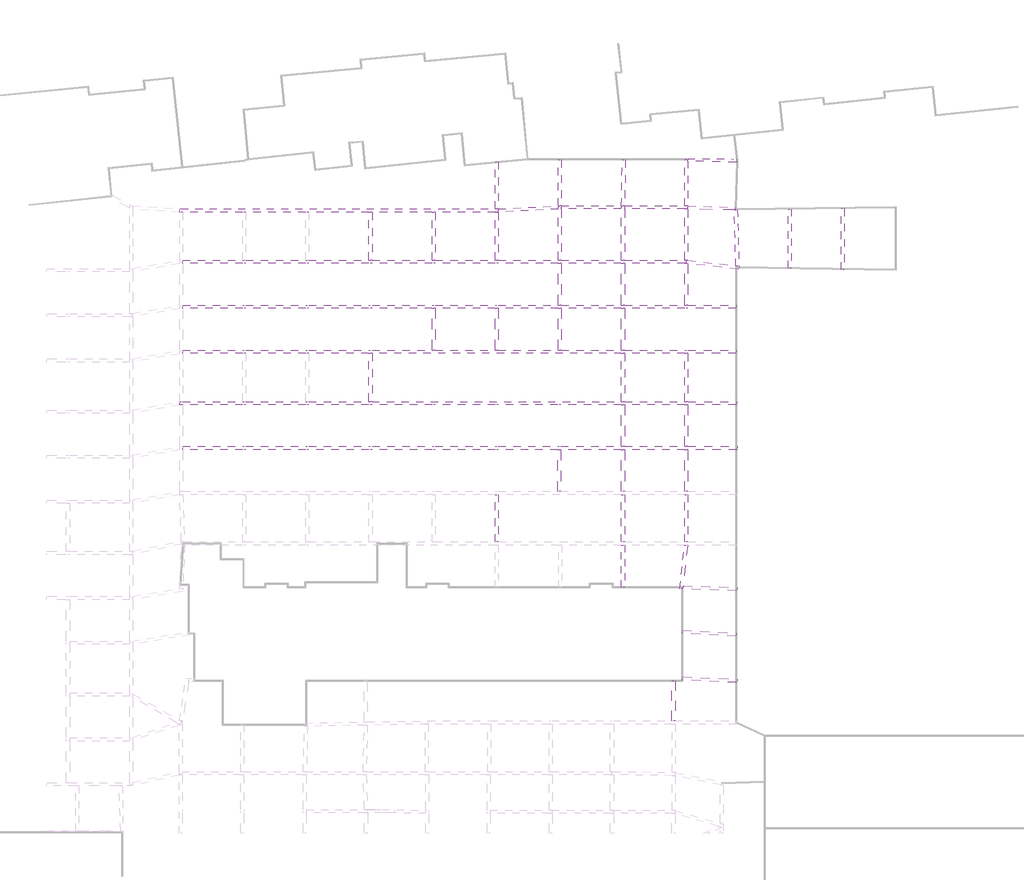
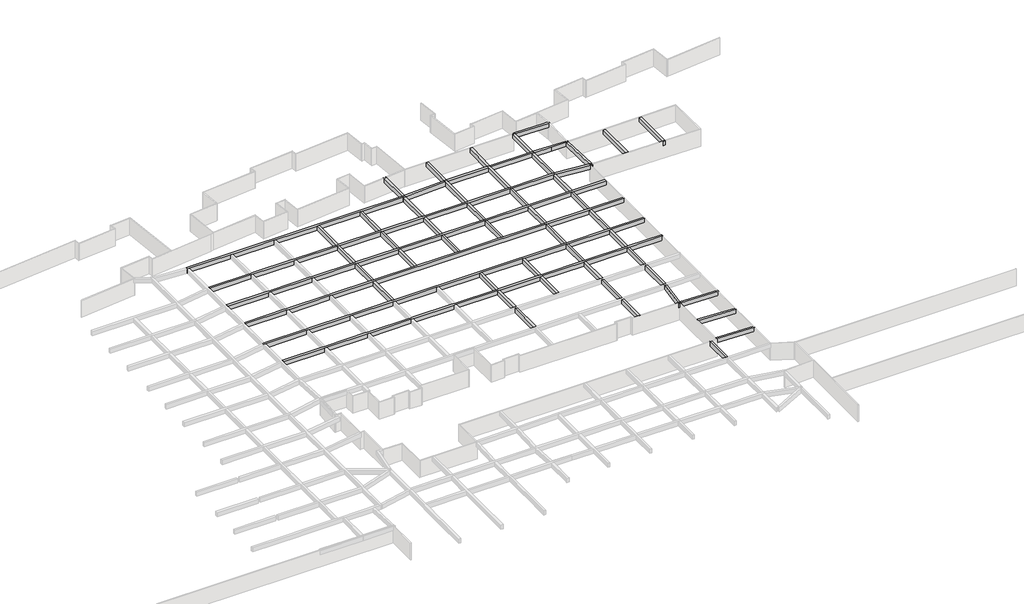
# One storey, part 20 of 20: 49 beams.
"""IFC4 building model written with IfcOpenShell, lengths in millimetres."""

import ifcopenshell
import ifcopenshell.guid

model = None  # the IFC model being written
_history = None  # IfcOwnerHistory: only IFC2X3 demands one
_inside = {}  # id of a spatial element -> (the spatial element, [elements in it])
_under = {}  # id of a project, library or spatial element -> (it, [spatial elements below it])
_declared = {}  # id of a project -> (the project, [libraries it declares])
_typed = {}  # id of a type object -> (the type object, [elements of that type])
_made_of = {}  # id of a material, layer set ... -> (it, [elements and type objects made of it])


def new_model(schema):
    """Start an empty IFC model of exactly this schema.

    Asked for "IFC4X3", IfcOpenShell would pick the latest addendum, in which some entities
    have other attributes; the version numbers below select the first issue.
    IFC2X3 requires an IfcOwnerHistory on every rooted entity: one is made here for all.
    """
    global model, _history
    if schema == "IFC4X3":
        model = ifcopenshell.file(schema_version=(4, 3, 0, 0))
    else:
        model = ifcopenshell.file(schema=schema)
    _inside.clear()
    _under.clear()
    _declared.clear()
    _typed.clear()
    _made_of.clear()
    _history = None
    if model.schema == "IFC2X3":
        org = make("IfcOrganization", Name="unknown")
        user = make(
            "IfcPersonAndOrganization",
            ThePerson=make("IfcPerson", FamilyName="unknown"),
            TheOrganization=org,
        )
        app = make(
            "IfcApplication",
            ApplicationDeveloper=org,
            Version="unknown",
            ApplicationFullName="unknown",
            ApplicationIdentifier="unknown",
        )
        _history = make(
            "IfcOwnerHistory",
            OwningUser=user,
            OwningApplication=app,
            ChangeAction="ADDED",
            CreationDate=0,
        )
    return model


def make(cls, **values):
    """One entity of the class cls with the attributes given. An attribute that is None is left unset."""
    return model.create_entity(
        cls, **{name: value for name, value in values.items() if value is not None}
    )


def rooted(cls, **values):
    """An entity with a GlobalId (a new one), such as an element, a storey or a relation."""
    return make(cls, GlobalId=ifcopenshell.guid.new(), OwnerHistory=_history, **values)


def si_unit(unit_type, name, prefix=None):
    """IfcSIUnit, for example si_unit("LENGTHUNIT", "METRE", prefix="MILLI")."""
    return make("IfcSIUnit", UnitType=unit_type, Prefix=prefix, Name=name)


def assignment(units):
    """IfcUnitAssignment: the units of a project."""
    return None if units is None else make("IfcUnitAssignment", Units=units)


def point(xyz):
    """IfcCartesianPoint."""
    return None if xyz is None else make("IfcCartesianPoint", Coordinates=xyz)


def direction(xyz):
    """IfcDirection."""
    return None if xyz is None else make("IfcDirection", DirectionRatios=xyz)


def frame(location, z_axis=None, x_axis=None):
    """IfcAxis2Placement3D, a coordinate frame: its origin and axes. An axis left out is left unset."""
    return make(
        "IfcAxis2Placement3D",
        Location=point(location),
        Axis=direction(z_axis),
        RefDirection=direction(x_axis),
    )


def origin():
    """The frame at (0, 0, 0) with its axes left unset."""
    return frame((0.0, 0.0, 0.0))


def place(relative_to, where):
    """IfcLocalPlacement: puts the frame where relative to a parent placement (None: the world)."""
    return make(
        "IfcLocalPlacement", PlacementRelTo=relative_to, RelativePlacement=where
    )


def context(
    kind, dimensions, precision=None, world=None, true_north=None, identifier=None
):
    """IfcGeometricRepresentationContext, for example the 3D "Model" context."""
    return make(
        "IfcGeometricRepresentationContext",
        ContextIdentifier=identifier,
        ContextType=kind,
        CoordinateSpaceDimension=dimensions,
        Precision=precision,
        WorldCoordinateSystem=world,
        TrueNorth=true_north,
    )


def project(units=None, contexts=None):
    """IfcProject with its units and contexts."""
    return rooted(
        "IfcProject",
        Name="project",
        RepresentationContexts=contexts,
        UnitsInContext=assignment(units),
    )


def spatial(cls, under=None, at=None, **own):
    """A site, building, storey or space (cls), placed at a placement, below another one or the project."""
    s = rooted(cls, ObjectPlacement=at, **own)
    if under is not None:
        _under.setdefault(under.id(), (under, []))[1].append(s)
    return s


def polyline(points):
    """IfcPolyline through the points."""
    return make("IfcPolyline", Points=[point(p) for p in points])


def outline(outer, holes=None, kind="AREA"):
    """IfcArbitraryClosedProfileDef: a profile drawn as a closed curve; with holes, ...WithVoids."""
    if holes is None:
        return make("IfcArbitraryClosedProfileDef", ProfileType=kind, OuterCurve=outer)
    return make(
        "IfcArbitraryProfileDefWithVoids",
        ProfileType=kind,
        OuterCurve=outer,
        InnerCurves=holes,
    )


def extrude(swept, where, along, depth):
    """IfcExtrudedAreaSolid: the profile swept, set in the frame where, extruded along a direction by depth."""
    return make(
        "IfcExtrudedAreaSolid",
        SweptArea=swept,
        Position=where,
        ExtrudedDirection=direction(along),
        Depth=depth,
    )


def faces_of(points, faces, orient=None, outer=None):
    """IfcFace entities. A face is a list of loops; a loop is a list of indices into points, from 0.

    orient and outer hold one flag for each loop. By default every Orientation is true, the
    first loop of a face is its IfcFaceOuterBound and the others are IfcFaceBound.
    """
    made = []
    for i, loops in enumerate(faces):
        bounds = []
        for j, loop in enumerate(loops):
            is_outer = j == 0 if outer is None else outer[i][j]
            bounds.append(
                make(
                    "IfcFaceOuterBound" if is_outer else "IfcFaceBound",
                    Bound=make("IfcPolyLoop", Polygon=[points[k] for k in loop]),
                    Orientation=True if orient is None else orient[i][j],
                )
            )
        made.append(make("IfcFace", Bounds=bounds))
    return made


def faceted_brep(points, faces, orient=None, outer=None, voids=None):
    """IfcFacetedBrep: a solid bounded by flat faces; with voids (closed shells), ...WithVoids."""
    shared = [point(p) for p in points]
    hull = make("IfcClosedShell", CfsFaces=faces_of(shared, faces, orient, outer))
    if voids is None:
        return make("IfcFacetedBrep", Outer=hull)
    return make(
        "IfcFacetedBrepWithVoids",
        Outer=hull,
        Voids=[
            make(cls, CfsFaces=faces_of(shared, fs, o, b)) for cls, fs, o, b in voids
        ],
    )


def shape(context_of_items, identifier, shape_type, items):
    """IfcShapeRepresentation: the items that make up one representation, for example the "Body"."""
    return make(
        "IfcShapeRepresentation",
        ContextOfItems=context_of_items,
        RepresentationIdentifier=identifier,
        RepresentationType=shape_type,
        Items=items,
    )


def source(mapping_origin, context_of_items, identifier, shape_type, items):
    """IfcRepresentationMap: a shape defined once, which mapped items show again and again."""
    return make(
        "IfcRepresentationMap",
        MappingOrigin=mapping_origin,
        MappedRepresentation=shape(context_of_items, identifier, shape_type, items),
    )


def transform(
    local_origin,
    x_axis=None,
    y_axis=None,
    z_axis=None,
    scale=None,
    scale2=None,
    scale3=None,
    uniform=True,
):
    """IfcCartesianTransformationOperator3D, or its non-uniform kind. x_axis, y_axis, z_axis: its Axis1, 2, 3."""
    if uniform:
        return make(
            "IfcCartesianTransformationOperator3D",
            Axis1=direction(x_axis),
            Axis2=direction(y_axis),
            LocalOrigin=point(local_origin),
            Scale=scale,
            Axis3=direction(z_axis),
        )
    return make(
        "IfcCartesianTransformationOperator3DnonUniform",
        Axis1=direction(x_axis),
        Axis2=direction(y_axis),
        LocalOrigin=point(local_origin),
        Scale=scale,
        Axis3=direction(z_axis),
        Scale2=scale2,
        Scale3=scale3,
    )


def mapped(mapping_source, mapping_target):
    """IfcMappedItem: shows the shape of a source again, moved by a transform."""
    return make(
        "IfcMappedItem", MappingSource=mapping_source, MappingTarget=mapping_target
    )


def made_of(thing, what):
    """Note that an element or type object is made of a material, layer set ...; save() writes the relation."""
    if what is not None:
        _made_of.setdefault(what.id(), (what, []))[1].append(thing)
    return thing


def element(
    cls,
    number,
    at=None,
    inside=None,
    cuts=None,
    type_object=None,
    material=None,
    context=None,
    identifier="Body",
    shape_type=None,
    held_by="IfcProductDefinitionShape",
    body=None,
    shapes=None,
    **own,
):
    """One element of the class cls, such as IfcWall. Its Tag is "e" and its number.

    at: its placement. inside: the storey or other place that contains it. cuts: it is an
    opening in that element (IfcRelVoidsElement). A single representation is given by context,
    identifier, shape_type and body (its items); several are given by shapes. held_by: the class
    of the entity that holds the representations. save() writes the other relations.
    """
    e = rooted(cls, Tag="e%d" % number, ObjectPlacement=at, **own)
    if body is not None:
        shapes = [shape(context, identifier, shape_type, body)]
    if shapes is not None:
        e.Representation = make(held_by, Representations=shapes)
    if inside is not None:
        _inside.setdefault(inside.id(), (inside, []))[1].append(e)
    if cuts is not None:
        rooted(
            "IfcRelVoidsElement", RelatingBuildingElement=cuts, RelatedOpeningElement=e
        )
    if type_object is not None:
        _typed.setdefault(type_object.id(), (type_object, []))[1].append(e)
    return made_of(e, material)


def aggregate(whole, parts):
    """IfcRelAggregates: a whole, such as a stair, and the parts it consists of."""
    return rooted("IfcRelAggregates", RelatingObject=whole, RelatedObjects=parts)


def save(model, path):
    """Write the relations noted so far, then the file.

    IfcRelAggregates (storeys below a building ...), IfcRelContainedInSpatialStructure (elements
    in a storey), IfcRelDefinesByType, IfcRelAssociatesMaterial and IfcRelDeclares: one each for
    every whole, place, type object, material and project.
    """
    for whole, parts in _under.values():
        aggregate(whole, parts)
    for where, things in _inside.values():
        rooted(
            "IfcRelContainedInSpatialStructure",
            RelatedElements=things,
            RelatingStructure=where,
        )
    for kind, things in _typed.values():
        rooted("IfcRelDefinesByType", RelatedObjects=things, RelatingType=kind)
    for what, things in _made_of.values():
        rooted("IfcRelAssociatesMaterial", RelatedObjects=things, RelatingMaterial=what)
    for by, libraries in _declared.values():
        rooted("IfcRelDeclares", RelatingContext=by, RelatedDefinitions=libraries)
    model.write(path)


def kl_beam_cbf95bda(model_context):
    return source(origin(), model_context, "Body", "SweptSolid", [
        extrude(outline(polyline([(3460.0, 200.0), (3460.0, -200.0), (-3460.0, -200.0), (-3460.0, 200.0), (3460.0, 200.0)])), frame((0.0, 0.0, -400.0), z_axis=(0.0, 0.0, 1.0), x_axis=(1.0, 0.0, 0.0)), (0.0, 0.0, 1.0), 800.0),
    ])


def kl_beam_04983839(model_context):
    return source(origin(), model_context, "Body", "SweptSolid", [
        extrude(outline(polyline([(3434.5, 200.0), (3434.5, -200.0), (-3434.5, -200.0), (-3434.5, 200.0), (3434.5, 200.0)])), frame((0.0, 0.0, -400.0), z_axis=(0.0, 0.0, 1.0), x_axis=(1.0, 0.0, 0.0)), (0.0, 0.0, 1.0), 800.0),
    ])


model = new_model("IFC4")

# Units and contexts
model_context = context("Model", 3, world=origin())
ifc_project = project(units=[si_unit("LENGTHUNIT", "METRE", prefix="MILLI")], contexts=[model_context])

# Site, building, storey
site = spatial("IfcSite", under=ifc_project)
building = spatial("IfcBuilding", under=site)
storey = spatial("IfcBuildingStorey", under=building, Name="户型图", Elevation=0.0)

# Beams
placement = place(None, origin())
element("IfcBeam", 1, ObjectType="混凝土 - 矩形梁 : KL_beam", at=placement, inside=storey, context=model_context, shape_type="SweptSolid", body=[
    extrude(outline(polyline([(171149.0, 132994.8835296), (171549.0, 132994.8835296), (171549.0, 127907.7670591), (171149.0, 127907.7670591), (171149.0, 132994.8835296)])), frame((0.0, 0.0, 2500.0), z_axis=(0.0, 0.0, 1.0), x_axis=(1.0, 0.0, 0.0)), (0.0, 0.0, 1.0), 800.0),
])
element("IfcBeam", 2, ObjectType="混凝土 - 矩形梁 : KL_beam", at=placement, inside=storey, context=model_context, shape_type="Brep", body=[
    faceted_brep([(179400.0, 162689.0, 3300.0), (179400.0, 162289.0, 3300.0), (179400.0, 162289.0, 2500.0), (179400.0, 162689.0, 2500.0), (173150.0, 162689.0, 3300.0), (172750.0, 162689.0, 3300.0), (165150.0, 162689.0, 3300.0), (164750.0, 162689.0, 3300.0), (157079.0, 162689.0, 3300.0), (156679.0, 162689.0, 3300.0), (149149.0, 162689.0, 3300.0), (148749.0, 162689.0, 3300.0), (141149.0, 162689.0, 3300.0), (140749.0, 162689.0, 3300.0), (133150.0, 162689.0, 3300.0), (132750.0, 162689.0, 3300.0), (125150.0, 162689.0, 3300.0), (124750.0, 162689.0, 3300.0), (117150.0, 162689.0, 3300.0), (116750.0, 162689.0, 3300.0), (109150.0, 162689.0, 3300.0), (109150.0, 162289.0, 3300.0), (116750.0, 162289.0, 3300.0), (117150.0, 162289.0, 3300.0), (124750.0, 162289.0, 3300.0), (125150.0, 162289.0, 3300.0), (132750.0, 162289.0, 3300.0), (133150.0, 162289.0, 3300.0), (140749.0, 162289.0, 3300.0), (141149.0, 162289.0, 3300.0), (148749.0, 162289.0, 3300.0), (149149.0, 162289.0, 3300.0), (156679.0, 162289.0, 3300.0), (157079.0, 162289.0, 3300.0), (164750.0, 162289.0, 3300.0), (165150.0, 162289.0, 3300.0), (172750.0, 162289.0, 3300.0), (173150.0, 162289.0, 3300.0), (109150.0, 162289.0, 2500.0), (116750.0, 162289.0, 2500.0), (117150.0, 162289.0, 2500.0), (124750.0, 162289.0, 2500.0), (125150.0, 162289.0, 2500.0), (132750.0, 162289.0, 2500.0), (133150.0, 162289.0, 2500.0), (140749.0, 162289.0, 2500.0), (141149.0, 162289.0, 2500.0), (148749.0, 162289.0, 2500.0), (149149.0, 162289.0, 2500.0), (156679.0, 162289.0, 2500.0), (157079.0, 162289.0, 2500.0), (164750.0, 162289.0, 2500.0), (165150.0, 162289.0, 2500.0), (172750.0, 162289.0, 2500.0), (173150.0, 162289.0, 2500.0), (109150.0, 162689.0, 2500.0), (116750.0, 162689.0, 2500.0), (117150.0, 162689.0, 2500.0), (124750.0, 162689.0, 2500.0), (125150.0, 162689.0, 2500.0), (132750.0, 162689.0, 2500.0), (133150.0, 162689.0, 2500.0), (140749.0, 162689.0, 2500.0), (141149.0, 162689.0, 2500.0), (148749.0, 162689.0, 2500.0), (149149.0, 162689.0, 2500.0), (156679.0, 162689.0, 2500.0), (157079.0, 162689.0, 2500.0), (164750.0, 162689.0, 2500.0), (165150.0, 162689.0, 2500.0), (172750.0, 162689.0, 2500.0), (173150.0, 162689.0, 2500.0)], [[[0, 1, 2, 3]], [[1, 0, 4, 5, 6, 7, 8, 9, 10, 11, 12, 13, 14, 15, 16, 17, 18, 19, 20, 21, 22, 23, 24, 25, 26, 27, 28, 29, 30, 31, 32, 33, 34, 35, 36, 37]], [[2, 1, 37, 36, 35, 34, 33, 32, 31, 30, 29, 28, 27, 26, 25, 24, 23, 22, 21, 38, 39, 40, 41, 42, 43, 44, 45, 46, 47, 48, 49, 50, 51, 52, 53, 54]], [[3, 2, 54, 53, 52, 51, 50, 49, 48, 47, 46, 45, 44, 43, 42, 41, 40, 39, 38, 55, 56, 57, 58, 59, 60, 61, 62, 63, 64, 65, 66, 67, 68, 69, 70, 71]], [[0, 3, 71, 70, 69, 68, 67, 66, 65, 64, 63, 62, 61, 60, 59, 58, 57, 56, 55, 20, 19, 18, 17, 16, 15, 14, 13, 12, 11, 10, 9, 8, 7, 6, 5, 4]], [[21, 20, 55, 38]]]),
])
element("IfcBeam", 3, ObjectType="混凝土 - 矩形梁 : KL_beam", at=placement, inside=storey, context=model_context, shape_type="Brep", body=[
    faceted_brep([(179350.0, 168389.0, 3300.0), (179350.0, 167989.0, 3300.0), (179350.0, 167989.0, 2500.0), (179350.0, 168389.0, 2500.0), (173150.0, 168389.0, 3300.0), (172750.0, 168389.0, 3300.0), (165150.0, 168389.0, 3300.0), (164750.0, 168389.0, 3300.0), (133150.0, 168389.0, 3300.0), (132750.0, 168389.0, 3300.0), (125150.0, 168389.0, 3300.0), (124750.0, 168389.0, 3300.0), (117150.0, 168389.0, 3300.0), (116750.0, 168389.0, 3300.0), (109150.0, 168389.0, 3300.0), (108750.0, 168389.0, 3300.0), (108750.0, 168357.1313923, 3300.0), (108750.0, 167989.0, 3300.0), (108967.3137137, 167989.0, 3300.0), (109150.0, 167989.0, 3300.0), (116750.0, 167989.0, 3300.0), (117150.0, 167989.0, 3300.0), (124750.0, 167989.0, 3300.0), (125150.0, 167989.0, 3300.0), (132750.0, 167989.0, 3300.0), (133150.0, 167989.0, 3300.0), (140749.0, 167989.0, 3300.0), (141149.0, 167989.0, 3300.0), (148749.0, 167989.0, 3300.0), (149149.0, 167989.0, 3300.0), (156679.0, 167989.0, 3300.0), (157079.0, 167989.0, 3300.0), (164750.0, 167989.0, 3300.0), (165150.0, 167989.0, 3300.0), (172750.0, 167989.0, 3300.0), (173150.0, 167989.0, 3300.0), (108750.0, 167989.0, 2500.0), (108967.3137137, 167989.0, 2500.0), (109150.0, 167989.0, 2500.0), (116750.0, 167989.0, 2500.0), (117150.0, 167989.0, 2500.0), (124750.0, 167989.0, 2500.0), (125150.0, 167989.0, 2500.0), (132750.0, 167989.0, 2500.0), (133150.0, 167989.0, 2500.0), (140749.0, 167989.0, 2500.0), (141149.0, 167989.0, 2500.0), (148749.0, 167989.0, 2500.0), (149149.0, 167989.0, 2500.0), (156679.0, 167989.0, 2500.0), (157079.0, 167989.0, 2500.0), (164750.0, 167989.0, 2500.0), (165150.0, 167989.0, 2500.0), (172750.0, 167989.0, 2500.0), (173150.0, 167989.0, 2500.0), (108750.0, 168357.1313923, 2500.0), (108750.0, 168389.0, 2500.0), (109150.0, 168389.0, 2500.0), (116750.0, 168389.0, 2500.0), (117150.0, 168389.0, 2500.0), (124750.0, 168389.0, 2500.0), (125150.0, 168389.0, 2500.0), (132750.0, 168389.0, 2500.0), (133150.0, 168389.0, 2500.0), (164750.0, 168389.0, 2500.0), (165150.0, 168389.0, 2500.0), (172750.0, 168389.0, 2500.0), (173150.0, 168389.0, 2500.0)], [[[0, 1, 2, 3]], [[1, 0, 4, 5, 6, 7, 8, 9, 10, 11, 12, 13, 14, 15, 16, 17, 18, 19, 20, 21, 22, 23, 24, 25, 26, 27, 28, 29, 30, 31, 32, 33, 34, 35]], [[2, 1, 35, 34, 33, 32, 31, 30, 29, 28, 27, 26, 25, 24, 23, 22, 21, 20, 19, 18, 17, 36, 37, 38, 39, 40, 41, 42, 43, 44, 45, 46, 47, 48, 49, 50, 51, 52, 53, 54]], [[3, 2, 54, 53, 52, 51, 50, 49, 48, 47, 46, 45, 44, 43, 42, 41, 40, 39, 38, 37, 36, 55, 56, 57, 58, 59, 60, 61, 62, 63, 64, 65, 66, 67]], [[0, 3, 67, 66, 65, 64, 63, 62, 61, 60, 59, 58, 57, 56, 15, 14, 13, 12, 11, 10, 9, 8, 7, 6, 5, 4]], [[17, 16, 15, 56, 55, 36]]]),
])
element("IfcBeam", 4, ObjectType="混凝土 - 矩形梁 : KL_beam", at=placement, inside=storey, context=model_context, shape_type="Brep", body=[
    faceted_brep([(179299.3844257, 174889.0, 3300.0), (179299.3844257, 174489.0, 3300.0), (179299.3844257, 174489.0, 2500.0), (179299.3844257, 174889.0, 2500.0), (173150.0, 174889.0, 3300.0), (172750.0, 174889.0, 3300.0), (165150.0, 174889.0, 3300.0), (164750.0, 174889.0, 3300.0), (157150.0, 174889.0, 3300.0), (156750.0, 174889.0, 3300.0), (149150.0, 174889.0, 3300.0), (148750.0, 174889.0, 3300.0), (141150.0, 174889.0, 3300.0), (140750.0, 174889.0, 3300.0), (133150.0, 174889.0, 3300.0), (132750.0, 174889.0, 3300.0), (125150.0, 174889.0, 3300.0), (124750.0, 174889.0, 3300.0), (117150.0, 174889.0, 3300.0), (116750.0, 174889.0, 3300.0), (109150.0, 174889.0, 3300.0), (109150.0, 174489.0, 3300.0), (116750.0, 174489.0, 3300.0), (117150.0, 174489.0, 3300.0), (124750.0, 174489.0, 3300.0), (125150.0, 174489.0, 3300.0), (132750.0, 174489.0, 3300.0), (133150.0, 174489.0, 3300.0), (164750.0, 174489.0, 3300.0), (165150.0, 174489.0, 3300.0), (172750.0, 174489.0, 3300.0), (173150.0, 174489.0, 3300.0), (109150.0, 174489.0, 2500.0), (116750.0, 174489.0, 2500.0), (117150.0, 174489.0, 2500.0), (124750.0, 174489.0, 2500.0), (125150.0, 174489.0, 2500.0), (132750.0, 174489.0, 2500.0), (133150.0, 174489.0, 2500.0), (164750.0, 174489.0, 2500.0), (165150.0, 174489.0, 2500.0), (172750.0, 174489.0, 2500.0), (173150.0, 174489.0, 2500.0), (109150.0, 174889.0, 2500.0), (116750.0, 174889.0, 2500.0), (117150.0, 174889.0, 2500.0), (124750.0, 174889.0, 2500.0), (125150.0, 174889.0, 2500.0), (132750.0, 174889.0, 2500.0), (133150.0, 174889.0, 2500.0), (140750.0, 174889.0, 2500.0), (141150.0, 174889.0, 2500.0), (148750.0, 174889.0, 2500.0), (149150.0, 174889.0, 2500.0), (156750.0, 174889.0, 2500.0), (157150.0, 174889.0, 2500.0), (164750.0, 174889.0, 2500.0), (165150.0, 174889.0, 2500.0), (172750.0, 174889.0, 2500.0), (173150.0, 174889.0, 2500.0)], [[[0, 1, 2, 3]], [[1, 0, 4, 5, 6, 7, 8, 9, 10, 11, 12, 13, 14, 15, 16, 17, 18, 19, 20, 21, 22, 23, 24, 25, 26, 27, 28, 29, 30, 31]], [[2, 1, 31, 30, 29, 28, 27, 26, 25, 24, 23, 22, 21, 32, 33, 34, 35, 36, 37, 38, 39, 40, 41, 42]], [[3, 2, 42, 41, 40, 39, 38, 37, 36, 35, 34, 33, 32, 43, 44, 45, 46, 47, 48, 49, 50, 51, 52, 53, 54, 55, 56, 57, 58, 59]], [[0, 3, 59, 58, 57, 56, 55, 54, 53, 52, 51, 50, 49, 48, 47, 46, 45, 44, 43, 20, 19, 18, 17, 16, 15, 14, 13, 12, 11, 10, 9, 8, 7, 6, 5, 4]], [[21, 20, 43, 32]]]),
])
element("IfcBeam", 5, ObjectType="混凝土 - 矩形梁 : KL_beam", at=placement, inside=storey, context=model_context, shape_type="Brep", body=[
    faceted_brep([(179299.3844257, 180590.0, 3300.0), (179299.3844257, 180190.0, 3300.0), (179299.3844257, 180190.0, 2500.0), (179299.3844257, 180590.0, 2500.0), (173150.0, 180590.0, 3300.0), (172750.0, 180590.0, 3300.0), (165150.0, 180590.0, 3300.0), (164750.0, 180590.0, 3300.0), (157150.0, 180590.0, 3300.0), (156750.0, 180590.0, 3300.0), (149150.0, 180590.0, 3300.0), (148750.0, 180590.0, 3300.0), (141150.0, 180590.0, 3300.0), (140750.0, 180590.0, 3300.0), (133150.0, 180590.0, 3300.0), (132750.0, 180590.0, 3300.0), (125150.0, 180590.0, 3300.0), (124750.0, 180590.0, 3300.0), (117150.0, 180590.0, 3300.0), (116750.0, 180590.0, 3300.0), (109150.0, 180590.0, 3300.0), (109150.0, 180190.0, 3300.0), (116750.0, 180190.0, 3300.0), (117150.0, 180190.0, 3300.0), (124750.0, 180190.0, 3300.0), (125150.0, 180190.0, 3300.0), (132750.0, 180190.0, 3300.0), (133150.0, 180190.0, 3300.0), (140750.0, 180190.0, 3300.0), (141150.0, 180190.0, 3300.0), (148750.0, 180190.0, 3300.0), (149150.0, 180190.0, 3300.0), (156750.0, 180190.0, 3300.0), (157150.0, 180190.0, 3300.0), (164750.0, 180190.0, 3300.0), (165150.0, 180190.0, 3300.0), (172750.0, 180190.0, 3300.0), (173150.0, 180190.0, 3300.0), (109150.0, 180190.0, 2500.0), (116750.0, 180190.0, 2500.0), (117150.0, 180190.0, 2500.0), (124750.0, 180190.0, 2500.0), (125150.0, 180190.0, 2500.0), (132750.0, 180190.0, 2500.0), (133150.0, 180190.0, 2500.0), (140750.0, 180190.0, 2500.0), (141150.0, 180190.0, 2500.0), (148750.0, 180190.0, 2500.0), (149150.0, 180190.0, 2500.0), (156750.0, 180190.0, 2500.0), (157150.0, 180190.0, 2500.0), (164750.0, 180190.0, 2500.0), (165150.0, 180190.0, 2500.0), (172750.0, 180190.0, 2500.0), (173150.0, 180190.0, 2500.0), (109150.0, 180590.0, 2500.0), (116750.0, 180590.0, 2500.0), (117150.0, 180590.0, 2500.0), (124750.0, 180590.0, 2500.0), (125150.0, 180590.0, 2500.0), (132750.0, 180590.0, 2500.0), (133150.0, 180590.0, 2500.0), (140750.0, 180590.0, 2500.0), (141150.0, 180590.0, 2500.0), (148750.0, 180590.0, 2500.0), (149150.0, 180590.0, 2500.0), (156750.0, 180590.0, 2500.0), (157150.0, 180590.0, 2500.0), (164750.0, 180590.0, 2500.0), (165150.0, 180590.0, 2500.0), (172750.0, 180590.0, 2500.0), (173150.0, 180590.0, 2500.0)], [[[0, 1, 2, 3]], [[1, 0, 4, 5, 6, 7, 8, 9, 10, 11, 12, 13, 14, 15, 16, 17, 18, 19, 20, 21, 22, 23, 24, 25, 26, 27, 28, 29, 30, 31, 32, 33, 34, 35, 36, 37]], [[2, 1, 37, 36, 35, 34, 33, 32, 31, 30, 29, 28, 27, 26, 25, 24, 23, 22, 21, 38, 39, 40, 41, 42, 43, 44, 45, 46, 47, 48, 49, 50, 51, 52, 53, 54]], [[3, 2, 54, 53, 52, 51, 50, 49, 48, 47, 46, 45, 44, 43, 42, 41, 40, 39, 38, 55, 56, 57, 58, 59, 60, 61, 62, 63, 64, 65, 66, 67, 68, 69, 70, 71]], [[0, 3, 71, 70, 69, 68, 67, 66, 65, 64, 63, 62, 61, 60, 59, 58, 57, 56, 55, 20, 19, 18, 17, 16, 15, 14, 13, 12, 11, 10, 9, 8, 7, 6, 5, 4]], [[21, 20, 55, 38]]]),
])
element("IfcBeam", 6, ObjectType="混凝土 - 矩形梁 : KL_beam", at=placement, inside=storey, context=model_context, shape_type="Brep", body=[
    faceted_brep([(172939.0529659, 185889.0, 3300.0), (172960.9470341, 186289.0, 3300.0), (172750.0, 186289.0, 3300.0), (165150.0, 186289.0, 3300.0), (164750.0, 186289.0, 3300.0), (157150.0, 186289.0, 3300.0), (156750.0, 186289.0, 3300.0), (149150.0, 186289.0, 3300.0), (148750.0, 186289.0, 3300.0), (141150.0, 186289.0, 3300.0), (140750.0, 186289.0, 3300.0), (133150.0, 186289.0, 3300.0), (132750.0, 186289.0, 3300.0), (125150.0, 186289.0, 3300.0), (124750.0, 186289.0, 3300.0), (117150.0, 186289.0, 3300.0), (116750.0, 186289.0, 3300.0), (109150.0, 186289.0, 3300.0), (109150.0, 185889.0, 3300.0), (116750.0, 185889.0, 3300.0), (117150.0, 185889.0, 3300.0), (124750.0, 185889.0, 3300.0), (125150.0, 185889.0, 3300.0), (132750.0, 185889.0, 3300.0), (133150.0, 185889.0, 3300.0), (140750.0, 185889.0, 3300.0), (141150.0, 185889.0, 3300.0), (148750.0, 185889.0, 3300.0), (149150.0, 185889.0, 3300.0), (156750.0, 185889.0, 3300.0), (157150.0, 185889.0, 3300.0), (164750.0, 185889.0, 3300.0), (165150.0, 185889.0, 3300.0), (172750.0, 185889.0, 3300.0), (172939.0529659, 185889.0, 2500.0), (109150.0, 185889.0, 2500.0), (116750.0, 185889.0, 2500.0), (117150.0, 185889.0, 2500.0), (124750.0, 185889.0, 2500.0), (125150.0, 185889.0, 2500.0), (132750.0, 185889.0, 2500.0), (133150.0, 185889.0, 2500.0), (140750.0, 185889.0, 2500.0), (141150.0, 185889.0, 2500.0), (148750.0, 185889.0, 2500.0), (149150.0, 185889.0, 2500.0), (156750.0, 185889.0, 2500.0), (157150.0, 185889.0, 2500.0), (164750.0, 185889.0, 2500.0), (165150.0, 185889.0, 2500.0), (172750.0, 185889.0, 2500.0), (172960.9470341, 186289.0, 2500.0), (109150.0, 186289.0, 2500.0), (116750.0, 186289.0, 2500.0), (117150.0, 186289.0, 2500.0), (124750.0, 186289.0, 2500.0), (125150.0, 186289.0, 2500.0), (132750.0, 186289.0, 2500.0), (133150.0, 186289.0, 2500.0), (140750.0, 186289.0, 2500.0), (141150.0, 186289.0, 2500.0), (148750.0, 186289.0, 2500.0), (149150.0, 186289.0, 2500.0), (156750.0, 186289.0, 2500.0), (157150.0, 186289.0, 2500.0), (164750.0, 186289.0, 2500.0), (165150.0, 186289.0, 2500.0), (172750.0, 186289.0, 2500.0)], [[[0, 1, 2, 3, 4, 5, 6, 7, 8, 9, 10, 11, 12, 13, 14, 15, 16, 17, 18, 19, 20, 21, 22, 23, 24, 25, 26, 27, 28, 29, 30, 31, 32, 33]], [[34, 0, 33, 32, 31, 30, 29, 28, 27, 26, 25, 24, 23, 22, 21, 20, 19, 18, 35, 36, 37, 38, 39, 40, 41, 42, 43, 44, 45, 46, 47, 48, 49, 50]], [[51, 34, 50, 49, 48, 47, 46, 45, 44, 43, 42, 41, 40, 39, 38, 37, 36, 35, 52, 53, 54, 55, 56, 57, 58, 59, 60, 61, 62, 63, 64, 65, 66, 67]], [[1, 51, 67, 66, 65, 64, 63, 62, 61, 60, 59, 58, 57, 56, 55, 54, 53, 52, 17, 16, 15, 14, 13, 12, 11, 10, 9, 8, 7, 6, 5, 4, 3, 2]], [[1, 0, 34, 51]], [[18, 17, 52, 35]]]),
])
element("IfcBeam", 7, ObjectType="混凝土 - 矩形梁 : KL_beam", at=placement, inside=storey, context=model_context, shape_type="Brep", body=[
    faceted_brep([(179648.9788512, 185554.6588326, 3300.0), (179247.6109832, 185598.7287409, 3300.0), (173150.0, 186268.2421179, 3300.0), (172960.9470341, 186289.0, 3300.0), (172939.0529659, 185889.0, 3300.0), (173150.0, 185865.8381647, 3300.0), (179605.3215094, 185157.0484247, 3300.0), (172939.0529659, 185889.0, 2500.0), (173150.0, 185865.8381647, 2500.0), (179605.3215094, 185157.0484247, 2500.0), (172960.9470341, 186289.0, 2500.0), (173150.0, 186268.2421179, 2500.0), (179247.6109832, 185598.7287409, 2500.0), (179648.9788512, 185554.6588326, 2500.0)], [[[0, 1, 2, 3, 4, 5, 6]], [[6, 5, 4, 7, 8, 9]], [[9, 8, 7, 10, 11, 12, 13]], [[3, 2, 1, 0, 13, 12, 11, 10]], [[3, 10, 7, 4]], [[0, 6, 9, 13]]]),
])
element("IfcBeam", 8, ObjectType="混凝土 - 矩形梁 : KL_beam", at=placement, inside=storey, context=model_context, shape_type="SweptSolid", body=[
    extrude(outline(polyline([(172750.0, 185889.0), (172939.0529659, 185889.0), (173150.0, 185865.8381647), (173150.0, 180590.0), (172750.0, 180590.0), (172750.0, 185889.0)])), frame((0.0, 0.0, 2500.0), z_axis=(0.0, 0.0, 1.0), x_axis=(1.0, 0.0, 0.0)), (0.0, 0.0, 1.0), 800.0),
])
element("IfcBeam", 9, ObjectType="混凝土 - 矩形梁 : KL_beam", at=placement, inside=storey, context=model_context, shape_type="SweptSolid", body=[
    extrude(outline(polyline([(165150.0, 180590.0), (164750.0, 180590.0), (164750.0, 185889.0), (165150.0, 185889.0), (165150.0, 180590.0)])), frame((0.0, 0.0, 2500.0), z_axis=(0.0, 0.0, 1.0), x_axis=(1.0, 0.0, 0.0)), (0.0, 0.0, 1.0), 800.0),
])
element("IfcBeam", 10, ObjectType="混凝土 - 矩形梁 : KL_beam", at=placement, inside=storey, context=model_context, shape_type="SweptSolid", body=[
    extrude(outline(polyline([(165150.0, 174889.0), (164750.0, 174889.0), (164750.0, 180190.0), (165150.0, 180190.0), (165150.0, 174889.0)])), frame((0.0, 0.0, 2500.0), z_axis=(0.0, 0.0, 1.0), x_axis=(1.0, 0.0, 0.0)), (0.0, 0.0, 1.0), 800.0),
])
element("IfcBeam", 11, ObjectType="混凝土 - 矩形梁 : KL_beam", at=placement, inside=storey, context=model_context, shape_type="SweptSolid", body=[
    extrude(outline(polyline([(165150.0, 168389.0), (164750.0, 168389.0), (164750.0, 174489.0), (165150.0, 174489.0), (165150.0, 168389.0)])), frame((0.0, 0.0, 2500.0), z_axis=(0.0, 0.0, 1.0), x_axis=(1.0, 0.0, 0.0)), (0.0, 0.0, 1.0), 800.0),
])
element("IfcBeam", 12, ObjectType="混凝土 - 矩形梁 : KL_beam", at=placement, inside=storey, context=model_context, shape_type="SweptSolid", body=[
    extrude(outline(polyline([(165150.0, 162689.0), (164750.0, 162689.0), (164750.0, 167989.0), (165150.0, 167989.0), (165150.0, 162689.0)])), frame((0.0, 0.0, 2500.0), z_axis=(0.0, 0.0, 1.0), x_axis=(1.0, 0.0, 0.0)), (0.0, 0.0, 1.0), 800.0),
])
element("IfcBeam", 13, ObjectType="混凝土 - 矩形梁 : KL_beam", at=placement, inside=storey, context=model_context, shape_type="SweptSolid", body=[
    extrude(outline(polyline([(165150.0, 156989.0), (164750.0, 156989.0), (164750.0, 162289.0), (165150.0, 162289.0), (165150.0, 156989.0)])), frame((0.0, 0.0, 2500.0), z_axis=(0.0, 0.0, 1.0), x_axis=(1.0, 0.0, 0.0)), (0.0, 0.0, 1.0), 800.0),
])
element("IfcBeam", 14, ObjectType="混凝土 - 矩形梁 : KL_beam", at=placement, inside=storey, context=model_context, shape_type="SweptSolid", body=[
    extrude(outline(polyline([(164750.0, 156589.0), (165150.0, 156589.0), (165150.0, 150597.0), (164750.0, 150597.0), (164750.0, 156589.0)])), frame((0.0, 0.0, 2500.0), z_axis=(0.0, 0.0, 1.0), x_axis=(1.0, 0.0, 0.0)), (0.0, 0.0, 1.0), 800.0),
])
element("IfcBeam", 15, ObjectType="混凝土 - 矩形梁 : KL_beam", at=placement, inside=storey, context=model_context, shape_type="SweptSolid", body=[
    extrude(outline(polyline([(172750.0, 156589.0), (173150.0, 156589.0), (173150.0, 150597.0), (172750.0, 150597.0), (172750.0, 156589.0)])), frame((0.0, 0.0, 2500.0), z_axis=(0.0, 0.0, 1.0), x_axis=(1.0, 0.0, 0.0)), (0.0, 0.0, 1.0), 800.0),
])
element("IfcBeam", 16, ObjectType="混凝土 - 矩形梁 : KL_beam", at=placement, inside=storey, context=model_context, shape_type="SweptSolid", body=[
    extrude(outline(polyline([(173150.0, 156989.0), (172750.0, 156989.0), (172750.0, 162289.0), (173150.0, 162289.0), (173150.0, 156989.0)])), frame((0.0, 0.0, 2500.0), z_axis=(0.0, 0.0, 1.0), x_axis=(1.0, 0.0, 0.0)), (0.0, 0.0, 1.0), 800.0),
])
element("IfcBeam", 17, ObjectType="混凝土 - 矩形梁 : KL_beam", at=placement, inside=storey, context=model_context, shape_type="SweptSolid", body=[
    extrude(outline(polyline([(173150.0, 162689.0), (172750.0, 162689.0), (172750.0, 167989.0), (173150.0, 167989.0), (173150.0, 162689.0)])), frame((0.0, 0.0, 2500.0), z_axis=(0.0, 0.0, 1.0), x_axis=(1.0, 0.0, 0.0)), (0.0, 0.0, 1.0), 800.0),
])
element("IfcBeam", 18, ObjectType="混凝土 - 矩形梁 : KL_beam", at=placement, inside=storey, context=model_context, shape_type="SweptSolid", body=[
    extrude(outline(polyline([(173150.0, 168389.0), (172750.0, 168389.0), (172750.0, 174489.0), (173150.0, 174489.0), (173150.0, 168389.0)])), frame((0.0, 0.0, 2500.0), z_axis=(0.0, 0.0, 1.0), x_axis=(1.0, 0.0, 0.0)), (0.0, 0.0, 1.0), 800.0),
    extrude(outline(polyline([(172750.0, 180190.0), (173150.0, 180190.0), (173150.0, 174889.0), (172750.0, 174889.0), (172750.0, 180190.0)])), frame((0.0, 0.0, 2500.0), z_axis=(0.0, 0.0, 1.0), x_axis=(1.0, 0.0, 0.0)), (0.0, 0.0, 1.0), 800.0),
])
element("IfcBeam", 19, ObjectType="混凝土 - 矩形梁 : KL_beam", at=placement, inside=storey, context=model_context, shape_type="SweptSolid", body=[
    extrude(outline(polyline([(157150.0, 180590.0), (156750.0, 180590.0), (156750.0, 185889.0), (157150.0, 185889.0), (157150.0, 180590.0)])), frame((0.0, 0.0, 2500.0), z_axis=(0.0, 0.0, 1.0), x_axis=(1.0, 0.0, 0.0)), (0.0, 0.0, 1.0), 800.0),
])
element("IfcBeam", 20, ObjectType="混凝土 - 矩形梁 : KL_beam", at=placement, inside=storey, context=model_context, shape_type="SweptSolid", body=[
    extrude(outline(polyline([(157150.0, 174889.0), (156750.0, 174889.0), (156750.0, 180190.0), (157150.0, 180190.0), (157150.0, 174889.0)])), frame((0.0, 0.0, 2500.0), z_axis=(0.0, 0.0, 1.0), x_axis=(1.0, 0.0, 0.0)), (0.0, 0.0, 1.0), 800.0),
])
element("IfcBeam", 21, ObjectType="混凝土 - 矩形梁 : KL_beam", at=placement, inside=storey, context=model_context, shape_type="Brep", body=[
    faceted_brep([(157150.0, 193189.0, 3300.0), (156750.0, 193189.0, 3300.0), (156750.0, 193179.2498439, 3300.0), (156750.0, 192778.7501561, 3300.0), (156750.0, 186289.0, 3300.0), (157150.0, 186289.0, 3300.0), (157150.0, 192789.0, 3300.0), (157150.0, 193189.0, 2500.0), (157150.0, 186289.0, 2500.0), (157150.0, 192789.0, 2500.0), (156750.0, 193189.0, 2500.0), (156750.0, 186289.0, 2500.0), (156750.0, 192778.7501561, 2500.0), (156750.0, 193179.2498439, 2500.0)], [[[0, 1, 2, 3, 4, 5, 6]], [[7, 0, 6, 5, 8, 9]], [[10, 7, 9, 8, 11, 12, 13]], [[1, 10, 13, 12, 11, 4, 3, 2]], [[5, 4, 11, 8]], [[1, 0, 7, 10]]]),
])
element("IfcBeam", 22, ObjectType="混凝土 - 矩形梁 : KL_beam", at=placement, inside=storey, context=model_context, shape_type="SweptSolid", body=[
    extrude(outline(polyline([(156750.0, 199007.0), (157150.0, 199007.0), (157150.0, 193189.0), (156750.0, 193189.0), (156750.0, 199007.0)])), frame((0.0, 0.0, 2500.0), z_axis=(0.0, 0.0, 1.0), x_axis=(1.0, 0.0, 0.0)), (0.0, 0.0, 1.0), 800.0),
])
element("IfcBeam", 23, ObjectType="混凝土 - 矩形梁 : KL_beam", at=placement, inside=storey, context=model_context, shape_type="Brep", body=[
    faceted_brep([(165150.0, 193189.0, 3300.0), (164753.4605474, 193189.0, 3300.0), (164750.0, 193189.0, 3300.0), (164750.0, 192789.0, 3300.0), (164750.0, 186289.0, 3300.0), (165150.0, 186289.0, 3300.0), (165150.0, 192789.0, 3300.0), (164750.0, 193189.0, 2500.0), (164750.0, 192789.0, 2500.0), (164750.0, 186289.0, 2500.0), (164753.4605474, 193189.0, 2500.0), (165150.0, 193189.0, 2500.0), (165150.0, 192789.0, 2500.0), (165150.0, 186289.0, 2500.0)], [[[0, 1, 2, 3, 4, 5, 6]], [[2, 7, 8, 9, 4, 3]], [[7, 10, 11, 12, 13, 9, 8]], [[11, 0, 6, 5, 13, 12]], [[5, 4, 9, 13]], [[2, 1, 0, 11, 10, 7]]]),
])
element("IfcBeam", 24, ObjectType="混凝土 - 矩形梁 : KL_beam", at=placement, inside=storey, context=model_context, shape_type="SweptSolid", body=[
    extrude(outline(polyline([(157150.0, 192789.0), (157150.0, 193189.0), (164750.0, 193189.0), (164750.0, 192789.0), (157150.0, 192789.0)])), frame((0.0, 0.0, 2500.0), z_axis=(0.0, 0.0, 1.0), x_axis=(1.0, 0.0, 0.0)), (0.0, 0.0, 1.0), 800.0),
])
element("IfcBeam", 25, ObjectType="混凝土 - 矩形梁 : KL_beam", at=placement, inside=storey, context=model_context, shape_type="Brep", body=[
    faceted_brep([(173150.0, 192789.0, 3300.0), (173150.0, 193182.0152687, 3300.0), (173150.0, 193189.0, 3300.0), (172750.0, 193189.0, 3300.0), (165153.5214786, 193189.0, 3300.0), (165150.0, 193189.0, 3300.0), (165150.0, 192789.0, 3300.0), (172750.0, 192789.0, 3300.0), (173150.0, 192789.0, 2500.0), (165150.0, 192789.0, 2500.0), (172750.0, 192789.0, 2500.0), (173150.0, 193189.0, 2500.0), (173150.0, 193182.0152687, 2500.0), (165150.0, 193189.0, 2500.0), (165153.5214786, 193189.0, 2500.0), (172750.0, 193189.0, 2500.0)], [[[0, 1, 2, 3, 4, 5, 6, 7]], [[8, 0, 7, 6, 9, 10]], [[11, 12, 8, 10, 9, 13, 14, 15]], [[2, 11, 15, 14, 13, 5, 4, 3]], [[6, 5, 13, 9]], [[2, 1, 0, 8, 12, 11]]]),
])
element("IfcBeam", 26, ObjectType="混凝土 - 矩形梁 : KL_beam", at=placement, inside=storey, context=model_context, shape_type="Brep", body=[
    faceted_brep([(172750.0, 186289.0, 3300.0), (172960.9470341, 186289.0, 3300.0), (173150.0, 186268.2421179, 3300.0), (173150.0, 192781.7625091, 3300.0), (173150.0, 192789.0, 3300.0), (172750.0, 192789.0, 3300.0), (172750.0, 186289.0, 2500.0), (172750.0, 192789.0, 2500.0), (172960.9470341, 186289.0, 2500.0), (173150.0, 192789.0, 2500.0), (173150.0, 192781.7625091, 2500.0), (173150.0, 186268.2421179, 2500.0)], [[[0, 1, 2, 3, 4, 5]], [[6, 0, 5, 7]], [[8, 6, 7, 9, 10, 11]], [[2, 11, 10, 9, 4, 3]], [[1, 0, 6, 8]], [[2, 1, 8, 11]], [[5, 4, 9, 7]]]),
])
element("IfcBeam", 27, ObjectType="混凝土 - 矩形梁 : KL_beam", at=placement, inside=storey, context=model_context, shape_type="Brep", body=[
    faceted_brep([(165255.0750463, 199007.0, 3300.0), (164855.0141151, 199007.0, 3300.0), (164753.4605474, 193189.0, 3300.0), (165150.0, 193189.0, 3300.0), (165153.5214786, 193189.0, 3300.0), (165255.0750463, 199007.0, 2500.0), (165153.5214786, 193189.0, 2500.0), (164855.0141151, 199007.0, 2500.0), (165150.0, 193189.0, 2500.0), (164753.4605474, 193189.0, 2500.0)], [[[0, 1, 2, 3, 4]], [[5, 0, 4, 6]], [[7, 5, 6, 8, 9]], [[1, 7, 9, 2]], [[1, 0, 5, 7]], [[2, 9, 8, 6, 4, 3]]]),
])
element("IfcBeam", 28, ObjectType="混凝土 - 矩形梁 : KL_beam", at=placement, inside=storey, context=model_context, shape_type="Brep", body=[
    faceted_brep([(173150.0, 199127.0, 3300.0), (172953.0, 199127.0, 3300.0), (172953.0, 199007.0, 3300.0), (172750.0, 199007.0, 3300.0), (172750.0, 193189.0, 3300.0), (173150.0, 193189.0, 3300.0), (173150.0, 198862.0420748, 3300.0), (173150.0, 199127.0, 2500.0), (173150.0, 193189.0, 2500.0), (173150.0, 198862.0420748, 2500.0), (172953.0, 199127.0, 2500.0), (172750.0, 193189.0, 2500.0), (172750.0, 199007.0, 2500.0), (172953.0, 199007.0, 2500.0)], [[[0, 1, 2, 3, 4, 5, 6]], [[7, 0, 6, 5, 8, 9]], [[10, 7, 9, 8, 11, 12, 13]], [[3, 12, 11, 4]], [[0, 7, 10, 1]], [[2, 13, 12, 3]], [[13, 2, 1, 10]], [[5, 4, 11, 8]]]),
])
element("IfcBeam", 29, ObjectType="混凝土 - 矩形梁 : KL_beam", at=placement, inside=storey, context=model_context, shape_type="Brep", body=[
    faceted_brep([(176247.3712236, 192671.6337545, 3300.0), (179051.6399641, 192702.792296, 3300.0), (179188.4957959, 192704.3129164, 3300.0), (179194.9310156, 192967.0843882, 3300.0), (173150.0, 193182.0152687, 3300.0), (173150.0, 192789.0, 3300.0), (173150.0, 192781.7625091, 3300.0), (176247.3712236, 192671.6337545, 2500.0), (173150.0, 192781.7625091, 2500.0), (179194.9310156, 192967.0843882, 2500.0), (179188.4957959, 192704.3129164, 2500.0), (179051.6399641, 192702.792296, 2500.0), (173150.0, 192789.0, 2500.0), (173150.0, 193182.0152687, 2500.0)], [[[0, 1, 2, 3, 4, 5, 6]], [[7, 0, 6, 8]], [[9, 10, 11, 7, 8, 12, 13]], [[13, 4, 3, 9]], [[0, 7, 11, 10, 2, 1]], [[2, 10, 9, 3]], [[4, 13, 12, 8, 6, 5]]]),
])
element("IfcBeam", 30, ObjectType="混凝土 - 矩形梁 : KL_beam", at=placement, inside=storey, context=model_context, shape_type="Brep", body=[
    faceted_brep([(179648.9788512, 185554.6588326, 3300.0), (179451.6695175, 192707.2370688, 3300.0), (179188.4957959, 192704.3129164, 3300.0), (179051.6399641, 192702.792296, 3300.0), (179247.6109832, 185598.7287409, 3300.0), (179247.6109832, 185598.7287409, 2500.0), (179051.6399641, 192702.792296, 2500.0), (179451.6695175, 192707.2370688, 2500.0), (179648.9788512, 185554.6588326, 2500.0), (179188.4957959, 192704.3129164, 2500.0)], [[[0, 1, 2, 3, 4]], [[5, 4, 3, 6]], [[7, 8, 5, 6, 9]], [[1, 0, 8, 7]], [[1, 7, 9, 6, 3, 2]], [[0, 4, 5, 8]]]),
    faceted_brep([(179444.7464565, 192958.2020614, 3300.0), (179444.7464565, 192958.2020614, 2500.0), (179314.862565, 192962.8201553, 2500.0), (179314.862565, 192962.8201553, 3300.0), (179448.3600359, 192827.207704, 2500.0), (179448.3600359, 192827.207704, 3300.0), (179311.5042041, 192825.6870836, 3300.0), (179311.5042041, 192825.6870836, 2500.0)], [[[0, 1, 2, 3]], [[4, 5, 6, 7]], [[1, 0, 5, 4]], [[6, 3, 2, 7]], [[5, 0, 3, 6]], [[1, 4, 7, 2]]]),
])
element("IfcBeam", 31, ObjectType="混凝土 - 矩形梁 : KL_beam", at=placement, inside=storey, context=model_context, shape_type="SweptSolid", body=[
    extrude(outline(polyline([(186299.2467742, 185290.6577884), (185899.2467742, 185290.6577884), (185899.2467742, 192778.8768161), (186299.2467742, 192783.3212606), (186299.2467742, 185290.6577884)])), frame((0.0, 0.0, 2500.0), z_axis=(0.0, 0.0, 1.0), x_axis=(1.0, 0.0, 0.0)), (0.0, 0.0, 1.0), 800.0),
])
element("IfcBeam", 32, ObjectType="混凝土 - 矩形梁 : KL_beam", at=placement, inside=storey, context=model_context, shape_type="SweptSolid", body=[
    extrude(outline(polyline([(193013.1702639, 185090.3509459), (192613.1702639, 185090.3509459), (192613.1702639, 192853.475966), (193013.1702639, 192857.9204105), (193013.1702639, 185090.3509459)])), frame((0.0, 0.0, 2500.0), z_axis=(0.0, 0.0, 1.0), x_axis=(1.0, 0.0, 0.0)), (0.0, 0.0, 1.0), 800.0),
])
element("IfcBeam", 33, ObjectType="混凝土 - 矩形梁 : KL_beam", at=placement, inside=storey, context=model_context, shape_type="SweptSolid", body=[
    extrude(outline(polyline([(179460.4210469, 198889.1384734), (179455.9754522, 198707.6100229), (179455.5515507, 198707.6204042), (179460.0770452, 198892.4114303), (179460.4210469, 198889.1384734)])), frame((0.0, 0.0, 2500.0), z_axis=(0.0, 0.0, 1.0), x_axis=(1.0, 0.0, 0.0)), (0.0, 0.0, 1.0), 800.0),
    extrude(outline(polyline([(178669.1152792, 199127.0), (179316.4259651, 199111.1474934), (179339.9229548, 198887.5885697), (179335.5875196, 198710.5582988), (173150.0, 198862.0420748), (173150.0, 199127.0), (178669.1152792, 199127.0)])), frame((0.0, 0.0, 2500.0), z_axis=(0.0, 0.0, 1.0), x_axis=(1.0, 0.0, 0.0)), (0.0, 0.0, 1.0), 800.0),
])
element("IfcBeam", 34, ObjectType="混凝土 - 矩形梁 : KL_beam", at=placement, inside=storey, context=model_context, shape_type="Brep", body=[
    faceted_brep([(149150.0, 192389.0, 3300.0), (149150.0, 192398.7501561, 3300.0), (149150.0, 192789.0, 3300.0), (148750.0, 192789.0, 3300.0), (108956.3428204, 192789.0, 3300.0), (108750.0, 192789.0, 3300.0), (108750.0, 192401.2956939, 3300.0), (108750.0, 192389.0, 3300.0), (109150.0, 192389.0, 3300.0), (116750.0, 192389.0, 3300.0), (117150.0, 192389.0, 3300.0), (124750.0, 192389.0, 3300.0), (125150.0, 192389.0, 3300.0), (132750.0, 192389.0, 3300.0), (133150.0, 192389.0, 3300.0), (140750.0, 192389.0, 3300.0), (141150.0, 192389.0, 3300.0), (148750.0, 192389.0, 3300.0), (148954.9968789, 192389.0, 3300.0), (149150.0, 192389.0, 2500.0), (108750.0, 192389.0, 2500.0), (109150.0, 192389.0, 2500.0), (116750.0, 192389.0, 2500.0), (117150.0, 192389.0, 2500.0), (124750.0, 192389.0, 2500.0), (125150.0, 192389.0, 2500.0), (132750.0, 192389.0, 2500.0), (133150.0, 192389.0, 2500.0), (140750.0, 192389.0, 2500.0), (141150.0, 192389.0, 2500.0), (148750.0, 192389.0, 2500.0), (148954.9968789, 192389.0, 2500.0), (149150.0, 192789.0, 2500.0), (149150.0, 192398.7501561, 2500.0), (108750.0, 192401.2956939, 2500.0), (108750.0, 192789.0, 2500.0), (108956.3428204, 192789.0, 2500.0), (148750.0, 192789.0, 2500.0)], [[[0, 1, 2, 3, 4, 5, 6, 7, 8, 9, 10, 11, 12, 13, 14, 15, 16, 17, 18]], [[19, 0, 18, 17, 16, 15, 14, 13, 12, 11, 10, 9, 8, 7, 20, 21, 22, 23, 24, 25, 26, 27, 28, 29, 30, 31]], [[32, 33, 19, 31, 30, 29, 28, 27, 26, 25, 24, 23, 22, 21, 20, 34, 35, 36, 37]], [[2, 32, 37, 36, 35, 5, 4, 3]], [[2, 1, 0, 19, 33, 32]], [[7, 6, 5, 35, 34, 20]]]),
])
element("IfcBeam", 35, ObjectType="混凝土 - 矩形梁 : KL_beam", at=placement, inside=storey, context=model_context, shape_type="Brep", body=[
    faceted_brep([(148750.0, 198789.0, 3300.0), (149150.0, 198789.0, 3300.0), (149150.0, 198789.0, 2500.0), (148750.0, 198789.0, 2500.0), (148750.0, 192789.0, 3300.0), (149150.0, 192789.0, 3300.0), (149150.0, 192799.2498439, 3300.0), (149150.0, 192789.0, 2500.0), (149150.0, 192799.2498439, 2500.0), (148750.0, 192789.0, 2500.0)], [[[0, 1, 2, 3]], [[1, 0, 4, 5, 6]], [[2, 1, 6, 5, 7, 8]], [[3, 2, 8, 7, 9]], [[0, 3, 9, 4]], [[5, 4, 9, 7]]]),
])
element("IfcBeam", 36, ObjectType="混凝土 - 矩形梁 : KL_beam", at=placement, inside=storey, context=model_context, shape_type="Brep", body=[
    faceted_brep([(156750.0, 192778.7501561, 2500.0), (156750.0, 192778.7501561, 3300.0), (149150.0, 192398.7501561, 3300.0), (149150.0, 192398.7501561, 2500.0), (156750.0, 192789.0, 2500.0), (156750.0, 193179.2498439, 2500.0), (156750.0, 193179.2498439, 3300.0), (156750.0, 192789.0, 3300.0), (149150.0, 192799.2498439, 3300.0), (149150.0, 192789.0, 3300.0), (149150.0, 192789.0, 2500.0), (149150.0, 192799.2498439, 2500.0)], [[[0, 1, 2, 3]], [[1, 0, 4, 5, 6, 7]], [[7, 6, 8, 9, 2, 1]], [[4, 0, 3, 10, 11, 5]], [[6, 5, 11, 8]], [[3, 2, 9, 8, 11, 10]]]),
    faceted_brep([(148750.0, 192378.7501561, 2500.0), (148750.0, 192378.7501561, 3300.0), (148750.0, 192389.0, 3300.0), (148750.0, 192389.0, 2500.0), (148954.9968789, 192389.0, 3300.0), (148954.9968789, 192389.0, 2500.0)], [[[0, 1, 2, 3]], [[4, 5, 3, 2]], [[1, 0, 5, 4]], [[1, 4, 2]], [[5, 0, 3]]]),
])
element("IfcBeam", 37, ObjectType="混凝土 - 矩形梁 : KL_beam", at=placement, inside=storey, context=model_context, shape_type="SweptSolid", body=[
    extrude(outline(polyline([(148954.9968789, 192389.0), (149150.0, 192389.0), (149150.0, 186289.0), (148750.0, 186289.0), (148750.0, 192378.7501561), (148954.9968789, 192389.0)])), frame((0.0, 0.0, 2500.0), z_axis=(0.0, 0.0, 1.0), x_axis=(1.0, 0.0, 0.0)), (0.0, 0.0, 1.0), 800.0),
    extrude(outline(polyline([(149150.0, 180590.0), (148750.0, 180590.0), (148750.0, 185889.0), (149150.0, 185889.0), (149150.0, 180590.0)])), frame((0.0, 0.0, 2500.0), z_axis=(0.0, 0.0, 1.0), x_axis=(1.0, 0.0, 0.0)), (0.0, 0.0, 1.0), 800.0),
])
element("IfcBeam", 38, ObjectType="混凝土 - 矩形梁 : KL_beam", at=placement, inside=storey, context=model_context, shape_type="SweptSolid", body=[
    extrude(outline(polyline([(140750.0, 192389.0), (141150.0, 192389.0), (141150.0, 186289.0), (140750.0, 186289.0), (140750.0, 192389.0)])), frame((0.0, 0.0, 2500.0), z_axis=(0.0, 0.0, 1.0), x_axis=(1.0, 0.0, 0.0)), (0.0, 0.0, 1.0), 800.0),
    extrude(outline(polyline([(141150.0, 180590.0), (140750.0, 180590.0), (140750.0, 185889.0), (141150.0, 185889.0), (141150.0, 180590.0)])), frame((0.0, 0.0, 2500.0), z_axis=(0.0, 0.0, 1.0), x_axis=(1.0, 0.0, 0.0)), (0.0, 0.0, 1.0), 800.0),
])
element("IfcBeam", 39, ObjectType="混凝土 - 矩形梁 : KL_beam", at=placement, inside=storey, context=model_context, shape_type="SweptSolid", body=[
    extrude(outline(polyline([(132750.0, 192389.0), (133150.0, 192389.0), (133150.0, 186289.0), (132750.0, 186289.0), (132750.0, 192389.0)])), frame((0.0, 0.0, 2500.0), z_axis=(0.0, 0.0, 1.0), x_axis=(1.0, 0.0, 0.0)), (0.0, 0.0, 1.0), 800.0),
    extrude(outline(polyline([(133150.0, 180590.0), (132750.0, 180590.0), (132750.0, 185889.0), (133150.0, 185889.0), (133150.0, 180590.0)])), frame((0.0, 0.0, 2500.0), z_axis=(0.0, 0.0, 1.0), x_axis=(1.0, 0.0, 0.0)), (0.0, 0.0, 1.0), 800.0),
])
element("IfcBeam", 40, ObjectType="混凝土 - 矩形梁 : KL_beam", at=placement, inside=storey, context=model_context, shape_type="SweptSolid", body=[
    extrude(outline(polyline([(132750.0, 180190.0), (133150.0, 180190.0), (133150.0, 174889.0), (132750.0, 174889.0), (132750.0, 180190.0)])), frame((0.0, 0.0, 2500.0), z_axis=(0.0, 0.0, 1.0), x_axis=(1.0, 0.0, 0.0)), (0.0, 0.0, 1.0), 800.0),
    extrude(outline(polyline([(133150.0, 168389.0), (132750.0, 168389.0), (132750.0, 174489.0), (133150.0, 174489.0), (133150.0, 168389.0)])), frame((0.0, 0.0, 2500.0), z_axis=(0.0, 0.0, 1.0), x_axis=(1.0, 0.0, 0.0)), (0.0, 0.0, 1.0), 800.0),
])
element("IfcBeam", 41, ObjectType="混凝土 - 矩形梁 : KL_beam", at=placement, inside=storey, context=model_context, shape_type="SweptSolid", body=[
    extrude(outline(polyline([(141150.0, 174889.0), (140750.0, 174889.0), (140750.0, 180190.0), (141150.0, 180190.0), (141150.0, 174889.0)])), frame((0.0, 0.0, 2500.0), z_axis=(0.0, 0.0, 1.0), x_axis=(1.0, 0.0, 0.0)), (0.0, 0.0, 1.0), 800.0),
])
element("IfcBeam", 42, ObjectType="混凝土 - 矩形梁 : KL_beam", at=placement, inside=storey, context=model_context, shape_type="SweptSolid", body=[
    extrude(outline(polyline([(149150.0, 174889.0), (148750.0, 174889.0), (148750.0, 180190.0), (149150.0, 180190.0), (149150.0, 174889.0)])), frame((0.0, 0.0, 2500.0), z_axis=(0.0, 0.0, 1.0), x_axis=(1.0, 0.0, 0.0)), (0.0, 0.0, 1.0), 800.0),
])
element("IfcBeam", 43, ObjectType="混凝土 - 矩形梁 : KL_beam", at=placement, inside=storey, context=model_context, shape_type="SweptSolid", body=[
    extrude(outline(polyline([(148749.0, 167989.0), (149149.0, 167989.0), (149149.0, 162689.0), (148749.0, 162689.0), (148749.0, 167989.0)])), frame((0.0, 0.0, 2500.0), z_axis=(0.0, 0.0, 1.0), x_axis=(1.0, 0.0, 0.0)), (0.0, 0.0, 1.0), 800.0),
    extrude(outline(polyline([(149149.0, 150597.0), (148749.0, 150597.0), (148749.0, 156589.0), (149149.0, 156589.0), (149149.0, 150597.0)])), frame((0.0, 0.0, 2500.0), z_axis=(0.0, 0.0, 1.0), x_axis=(1.0, 0.0, 0.0)), (0.0, 0.0, 1.0), 800.0),
    extrude(outline(polyline([(149149.0, 156989.0), (148749.0, 156989.0), (148749.0, 162289.0), (149149.0, 162289.0), (149149.0, 156989.0)])), frame((0.0, 0.0, 2500.0), z_axis=(0.0, 0.0, 1.0), x_axis=(1.0, 0.0, 0.0)), (0.0, 0.0, 1.0), 800.0),
])
element("IfcBeam", 44, ObjectType="混凝土 - 矩形梁 : KL_beam", at=placement, inside=storey, context=model_context, shape_type="SweptSolid", body=[
    extrude(outline(polyline([(156679.0, 167989.0), (157079.0, 167989.0), (157079.0, 162689.0), (156679.0, 162689.0), (156679.0, 167989.0)])), frame((0.0, 0.0, 2500.0), z_axis=(0.0, 0.0, 1.0), x_axis=(1.0, 0.0, 0.0)), (0.0, 0.0, 1.0), 800.0),
    extrude(outline(polyline([(157079.0, 156989.0), (156679.0, 156989.0), (156679.0, 162289.0), (157079.0, 162289.0), (157079.0, 156989.0)])), frame((0.0, 0.0, 2500.0), z_axis=(0.0, 0.0, 1.0), x_axis=(1.0, 0.0, 0.0)), (0.0, 0.0, 1.0), 800.0),
])
element("IfcBeam", 45, ObjectType="混凝土 - 矩形梁 : KL_beam", at=placement, inside=storey, context=model_context, shape_type="SweptSolid", body=[
    extrude(outline(polyline([(165150.0, 144848.0), (164750.0, 144848.0), (164750.0, 150197.0), (165150.0, 150197.0), (165150.0, 144848.0)])), frame((0.0, 0.0, 2500.0), z_axis=(0.0, 0.0, 1.0), x_axis=(1.0, 0.0, 0.0)), (0.0, 0.0, 1.0), 800.0),
])
element("IfcBeam", 46, ObjectType="混凝土 - 矩形梁 : KL_beam", at=placement, inside=storey, context=model_context, shape_type="Brep", body=[
    faceted_brep([(172148.6411185, 144685.9339897, 3300.0), (172546.4498767, 144644.1226044, 3300.0), (172588.3633611, 145042.902771, 3300.0), (173130.0808089, 150197.0, 3300.0), (172727.877497, 150197.0, 3300.0), (172148.6411185, 144685.9339897, 2500.0), (172727.877497, 150197.0, 2500.0), (172546.4498767, 144644.1226044, 2500.0), (173130.0808089, 150197.0, 2500.0), (172588.3633611, 145042.902771, 2500.0)], [[[0, 1, 2, 3, 4]], [[5, 0, 4, 6]], [[7, 5, 6, 8, 9]], [[1, 7, 9, 8, 3, 2]], [[4, 3, 8, 6]], [[1, 0, 5, 7]]]),
])
element("IfcBeam", 47, ObjectType="混凝土 - 矩形梁 : KL_beam", at=placement, inside=storey, context=model_context, shape_type="Brep", body=[
    faceted_brep([(179406.8567099, 144804.7957365, 3300.0), (179392.8969112, 144405.0394057, 3300.0), (179392.8969112, 144405.0394057, 2500.0), (179406.8567099, 144804.7957365, 2500.0), (172588.3633611, 145042.902771, 3300.0), (172546.4498767, 144644.1226044, 3300.0), (172145.7173816, 144658.1164915, 3300.0), (172145.7173816, 144658.1164915, 2500.0), (172546.4498767, 144644.1226044, 2500.0), (172588.3633611, 145042.902771, 2500.0), (172148.6411185, 144685.9339897, 3300.0), (172148.6411185, 144685.9339897, 2500.0)], [[[0, 1, 2, 3]], [[1, 0, 4, 5]], [[2, 1, 5, 6, 7, 8]], [[3, 2, 8, 9]], [[0, 3, 9, 4]], [[7, 6, 10, 11]], [[8, 5, 4, 9]], [[5, 8, 11, 10]], [[10, 6, 5]], [[8, 7, 11]]]),
])
kl_beam_shape = kl_beam_cbf95bda(model_context)
element("IfcBeam", 48, ObjectType="混凝土 - 矩形梁 : KL_beam", at=placement, inside=storey, context=model_context, shape_type="MappedRepresentation", body=[
    mapped(kl_beam_shape, transform((175943.0836812, 133136.0464472, 2900.0), x_axis=(-0.9991087626622469, 0.04220995583406518, 0.0), y_axis=(-0.04220995583406518, -0.9991087626622469, 0.0), z_axis=(0.0, 0.0, 1.0))),
])
kl_beam_2_shape = kl_beam_04983839(model_context)
element("IfcBeam", 49, ObjectType="混凝土 - 矩形梁 : KL_beam", at=placement, inside=storey, context=model_context, shape_type="MappedRepresentation", body=[
    mapped(kl_beam_2_shape, transform((175869.8844257, 139032.752626, 2900.0), x_axis=(-0.9986295347545737, 0.052335956242946985, 0.0), y_axis=(-0.052335956242946985, -0.9986295347545737, 0.0), z_axis=(0.0, 0.0, 1.0))),
])

save(model, "model.ifc")

# Revit data of these elements
# Type "混凝土 - 矩形梁 : KL_beam"
#   Length [instance default] = 1524 mm
#   b = 400 mm
#   h = 800 mm
#   Structural Material [instance default] = 混凝土 - 现场浇注混凝土
#   Assembly Code = ""
# Elements 1, 2, 3, 4, 5, 6, 7, 8, 9, 10, 11, 12, 13, 14, 15, 16, 17, 18, 19, 20, 21, 22, 23, 24, 25, 26, 27, 28, 29, 30, 31, 32, 33, 34, 35, 36, 37, 38, 39, 40, 41, 42, 43, 44, 45, 46, 47, 48, 49 (IfcBeam, "混凝土 - 矩形梁 : KL_beam")
#   Comments = ""
#   Structural Material = none
#   Phase Created = 新构造
# Materials
#   "混凝土 - 现场浇注混凝土": class "混凝土", colour RGB 192 192 192, transparency 0
